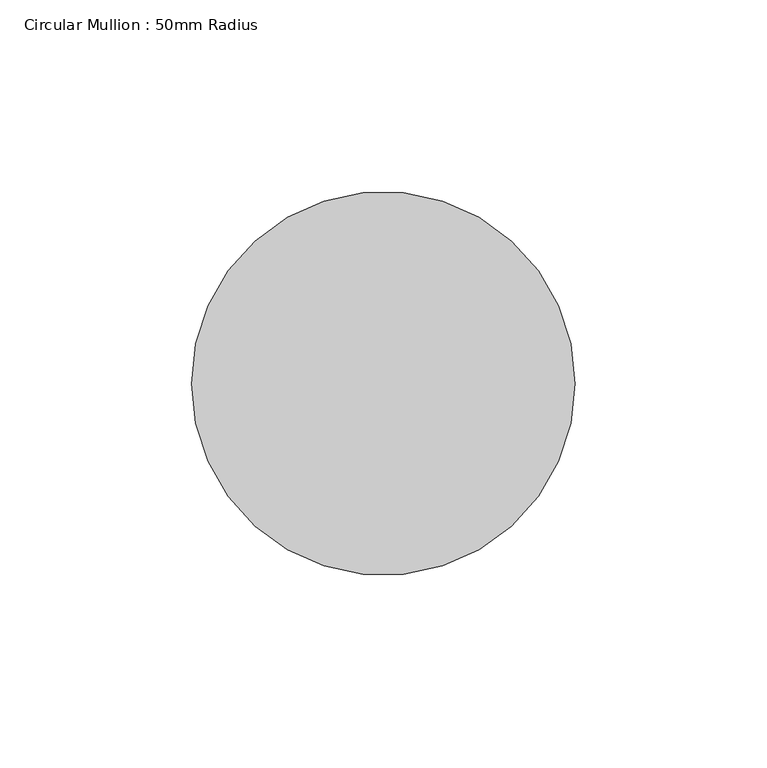
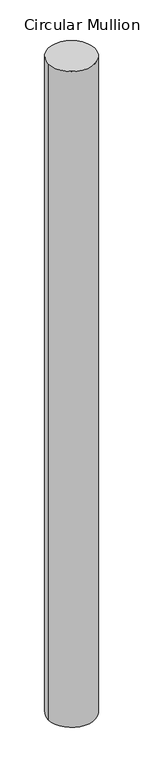
"""IFC4 building model written with IfcOpenShell, lengths in millimetres: member geometry, Circular Mullion : 50mm Radius."""

from ifc_helpers import new_model, si_unit, point, frame, origin, origin_2d, place, context, project, spatial, circle_curve, trimmed, segment, composite_curve, outline, extrude, source, transform, mapped, element, save


def circular_mullion_50mm_radius_381468fd(model_context):
    return source(origin(), model_context, "Body", "SweptSolid", [
        extrude(outline(composite_curve([segment(trimmed(circle_curve(origin_2d(), 50.0), [point((50.0, 0.0))], [point((-50.0, 0.0))], False, "CARTESIAN"), True, "CONTINUOUS"), segment(trimmed(circle_curve(origin_2d(), 50.0), [point((-50.0, 0.0))], [point((50.0, 0.0))], False, "CARTESIAN"), True, "CONTINUOUS")], self_intersect=False)), frame((0.0, 0.0, -1484.5544672), z_axis=(0.0, 0.0, 1.0), x_axis=(1.0, 0.0, 0.0)), (0.0, 0.0, 1.0), 1484.5544672),
    ])


if __name__ == "__main__":
    model = new_model("IFC4")
    model_context = context("Model", 3, world=origin())
    ifc_project = project(units=[si_unit("LENGTHUNIT", "METRE", prefix="MILLI")], contexts=[model_context])
    site = spatial("IfcSite", under=ifc_project)
    building = spatial("IfcBuilding", under=site)
    placement = place(None, origin())
    circular_mullion_50mm_radius_shape = circular_mullion_50mm_radius_381468fd(model_context)
    element("IfcMember", 1, ObjectType="Circular Mullion : 50mm Radius", at=placement, inside=building, context=model_context, shape_type="MappedRepresentation", body=[
        mapped(circular_mullion_50mm_radius_shape, transform((0.0, 0.0, 0.0), x_axis=(1.0, 0.0, 0.0), y_axis=(0.0, 1.0, 0.0), z_axis=(0.0, 0.0, 1.0))),
    ])
    save(model, "model.ifc")

# Revit data of these elements
# Type "Circular Mullion : 50mm Radius"
#   built-in parameter 1007350 = 0.164042 (stored number, unit not read)
# Element 1 (IfcMember, "Circular Mullion : 50mm Radius")
#   Materials on its faces: "Aluminium"
# Materials
#   "Aluminium": class "Metal", colour RGB 247 247 247, transparency 0, Description = "Aluminium 6061", Cost = 0
